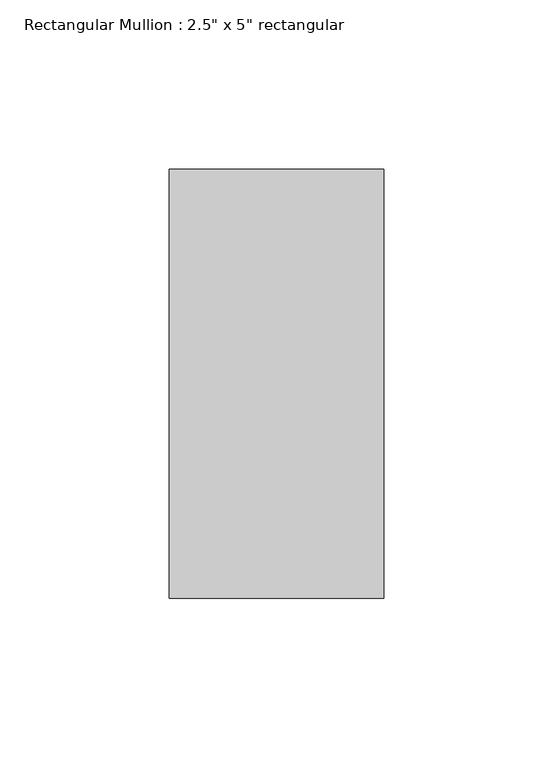
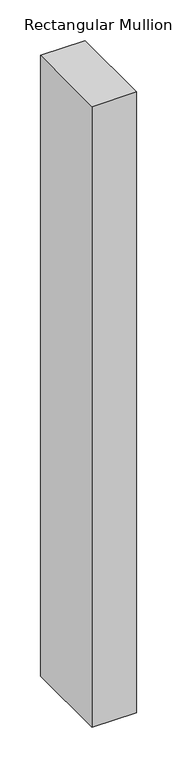
"""IFC4 building model written with IfcOpenShell, lengths in millimetres: member geometry."""

from ifc_helpers import new_model, si_unit, frame, origin, place, context, project, spatial, polyline, outline, extrude, source, transform, mapped, element, save


def member_03f32644(model_context):
    return source(origin(), model_context, "Body", "SweptSolid", [
        extrude(outline(polyline([(0.0, 63.5), (0.0, -63.5), (-63.5, -63.5), (-63.5, 63.5), (0.0, 63.5)])), frame((0.0, 0.0, -933.4500001), z_axis=(0.0, 0.0, 1.0), x_axis=(1.0, 0.0, 0.0)), (0.0, 0.0, 1.0), 933.4500001),
    ])


if __name__ == "__main__":
    model = new_model("IFC4")
    model_context = context("Model", 3, world=origin())
    ifc_project = project(units=[si_unit("LENGTHUNIT", "METRE", prefix="MILLI")], contexts=[model_context])
    site = spatial("IfcSite", under=ifc_project)
    building = spatial("IfcBuilding", under=site)
    placement = place(None, origin())
    member_shape = member_03f32644(model_context)
    element("IfcMember", 1, ObjectType="Rectangular Mullion : 2.5\" x 5\" rectangular", at=placement, inside=building, context=model_context, shape_type="MappedRepresentation", body=[
        mapped(member_shape, transform((0.0, 0.0, 0.0), x_axis=(1.0, 0.0, 0.0), y_axis=(0.0, 1.0, 0.0), z_axis=(0.0, 0.0, 1.0))),
    ])
    save(model, "model.ifc")

# Revit data of these elements
# Type "Rectangular Mullion : 2.5\" x 5\" rectangular"
#   built-in parameter 1007304 = 0.416667 (stored number, unit not read)
#   built-in parameter 1007301 = 0.104167 (stored number, unit not read)
#   built-in parameter 1007300 = 0.104167 (stored number, unit not read)
# Element 1 (IfcMember, "Rectangular Mullion : 2.5\" x 5\" rectangular")
#   Materials on its faces: "Aluminum"
# Materials
#   "Aluminum": class "Metal", colour RGB 247 247 247, transparency 0, Description = "Aluminum 6061", Cost = 0
